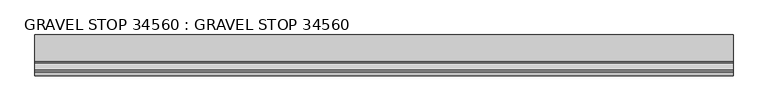
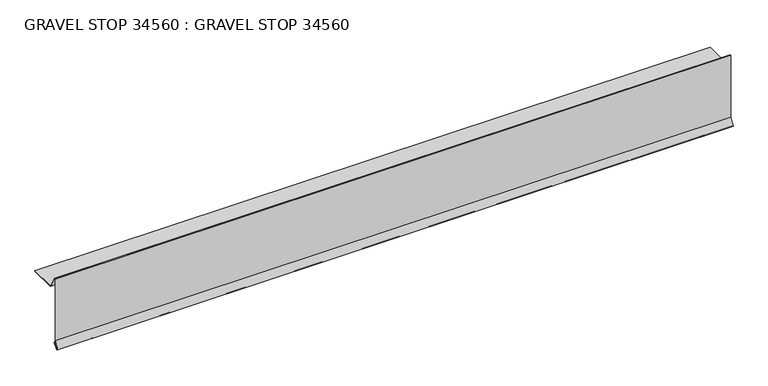
"""IFC4 building model written with IfcOpenShell, lengths in millimetres: proxy geometry, GRAVEL STOP 34560 : GRAVEL STOP 34560."""

from ifc_helpers import new_model, si_unit, frame, origin, place, context, project, spatial, polyline, outline, extrude, source, transform, mapped, element, save


def gravel_stop_34560_gravel_stop_34560_d8bdad0e(model_context):
    return source(origin(), model_context, "Body", "SweptSolid", [
        extrude(outline(polyline([(-5587.6106629, 40061.0736754), (-5591.684607, 40064.1815506), (-5580.0356381, 40085.5191254), (-5580.0356381, 40278.1940248), (-5577.0037237, 40279.0064238), (-5556.3332702, 40243.204148), (-5552.58096, 40241.0377507), (-5475.1230533, 40241.0377507), (-5475.1230533, 40239.6266397), (-5552.959066, 40239.6266397), (-5557.3662751, 40242.1711431), (-5577.6843899, 40277.3631503), (-5578.6245271, 40277.1112413), (-5578.6245271, 40085.1590213), (-5589.8655469, 40064.5686925), (-5587.7358967, 40062.9440538), (-5574.2139721, 40076.4659785), (-5573.2161659, 40075.4681723), (-5587.6106629, 40061.0736754)])), frame((12382.7678845, 0.0, 0.0), z_axis=(1.0, 0.0, 0.0), x_axis=(0.0, 1.0, 0.0)), (0.0, 0.0, 1.0), 2000.25),
    ])


if __name__ == "__main__":
    model = new_model("IFC4")
    model_context = context("Model", 3, world=origin())
    ifc_project = project(units=[si_unit("LENGTHUNIT", "METRE", prefix="MILLI")], contexts=[model_context])
    site = spatial("IfcSite", under=ifc_project)
    building = spatial("IfcBuilding", under=site)
    placement = place(None, origin())
    gravel_stop_34560_gravel_stop_34560_shape = gravel_stop_34560_gravel_stop_34560_d8bdad0e(model_context)
    element("IfcBuildingElementProxy", 1, Name="GRAVEL STOP 34560 : GRAVEL STOP 34560", ObjectType="GRAVEL STOP 34560 : GRAVEL STOP 34560", at=placement, inside=building, context=model_context, shape_type="MappedRepresentation", body=[
        mapped(gravel_stop_34560_gravel_stop_34560_shape, transform((0.0, 0.0, 0.0), x_axis=(1.0, 0.0, 0.0), y_axis=(0.0, 1.0, 0.0), z_axis=(0.0, 0.0, 1.0))),
    ])
    save(model, "model.ifc")

# Revit data of these elements
# Type "GRAVEL STOP 34560 : GRAVEL STOP 34560"
#   NameOverride = "GRAVEL STOP"
# Element 1 (IfcBuildingElementProxy, "GRAVEL STOP 34560 : GRAVEL STOP 34560")
#   Materials on its faces: "GRAVEL STOP REQUIRED WITH GRAVEL SURFACE SYSTEMS"
# Materials
#   "GRAVEL STOP REQUIRED WITH GRAVEL SURFACE SYSTEMS": class "Unassigned", colour RGB 170 170 127, transparency 0
